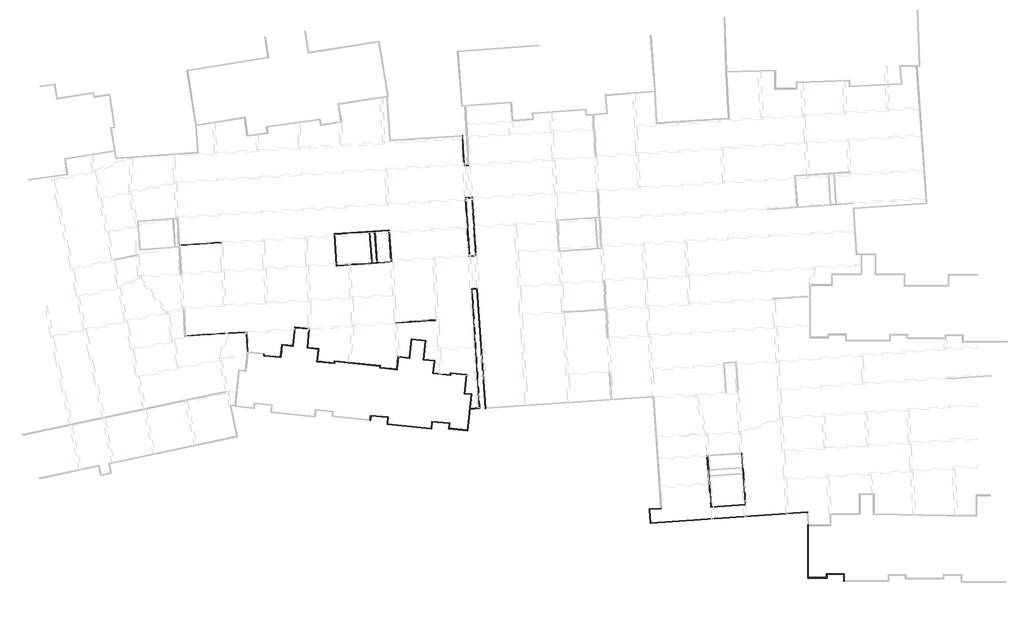
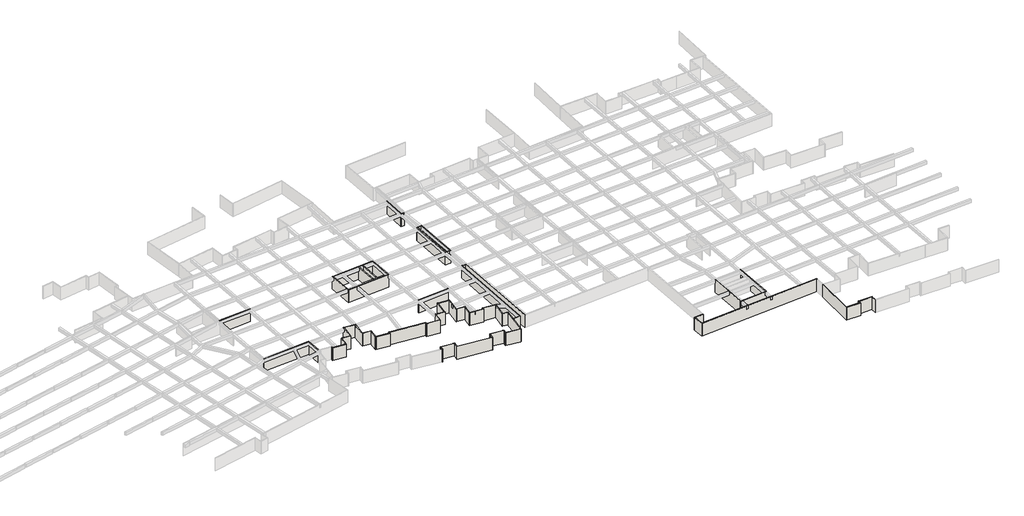
# One storey, part 4 of 14: 66 walls.
"""IFC4 building model written with IfcOpenShell, lengths in millimetres."""

from ifc_helpers import new_model, si_unit, origin, origin_with_axes, place, context, project, spatial, polyline, outline, extrude, faceted_brep, element, save

model = new_model("IFC4")

# Units and contexts
model_context = context("Model", 3, world=origin())
ifc_project = project(units=[si_unit("LENGTHUNIT", "METRE", prefix="MILLI")], contexts=[model_context])

# Site, building, storey
site = spatial("IfcSite", under=ifc_project)
building = spatial("IfcBuilding", under=site)
storey = spatial("IfcBuildingStorey", under=building, Name="户型图", Elevation=0.0)

# Walls
placement = place(None, origin())
element("IfcWall", 1, ObjectType="所有墙体", at=placement, inside=storey, context=model_context, shape_type="Brep", body=[
    faceted_brep([(-177282.9502682, -168363.1803001, 0.0), (-177324.8720819, -168762.0397145, 0.0), (-177324.8720819, -168762.0397145, 3300.0), (-177282.9502682, -168363.1803001, 3300.0), (-177163.6076407, -168375.7237157, 0.0), (-177163.6076407, -168375.7237157, 3300.0), (-177192.765182, -168653.1391901, 3300.0), (-177205.3105083, -168772.4999968, 3300.0), (-177205.3105083, -168772.4999968, 0.0), (-177192.765182, -168653.1391901, 0.0)], [[[0, 1, 2, 3]], [[4, 5, 6, 7, 8, 9]], [[1, 0, 4, 9, 8]], [[3, 2, 7, 6, 5]], [[0, 3, 5, 4]], [[2, 1, 8, 7]]]),
])
element("IfcWall", 2, ObjectType="所有墙体", at=placement, inside=storey, context=model_context, shape_type="Brep", body=[
    faceted_brep([(-177205.3105083, -168772.4999968, 0.0), (-174017.4874744, -169051.3983736, 0.0), (-174017.4874744, -169051.3983736, 3300.0), (-177205.3105083, -168772.4999968, 3300.0), (-177192.765182, -168653.1391901, 0.0), (-177192.765182, -168653.1391901, 3300.0), (-174124.5037217, -168921.5772846, 3300.0), (-174004.9421481, -168932.0375669, 3300.0), (-174004.9421481, -168932.0375669, 0.0), (-174124.5037217, -168921.5772846, 0.0)], [[[0, 1, 2, 3]], [[4, 5, 6, 7, 8, 9]], [[1, 0, 4, 9, 8]], [[3, 2, 7, 6, 5]], [[0, 3, 5, 4]], [[2, 1, 8, 7]]]),
])
element("IfcWall", 3, ObjectType="所有墙体", at=placement, inside=storey, context=model_context, shape_type="Brep", body=[
    faceted_brep([(-174004.9421481, -168932.0375669, 0.0), (-173766.7276803, -166665.5783017, 0.0), (-173754.1842647, -166546.2356743, 0.0), (-173754.1842647, -166546.2356743, 3300.0), (-173766.7276803, -166665.5783017, 3300.0), (-174004.9421481, -168932.0375669, 3300.0), (-174124.5037217, -168921.5772846, 0.0), (-174124.5037217, -168921.5772846, 3300.0), (-173873.5268921, -166533.6922587, 3300.0), (-173873.5268921, -166533.6922587, 0.0)], [[[0, 1, 2, 3, 4, 5]], [[6, 7, 8, 9]], [[2, 1, 0, 6, 9]], [[5, 4, 3, 8, 7]], [[0, 5, 7, 6]], [[3, 2, 9, 8]]]),
])
element("IfcWall", 4, ObjectType="所有墙体", at=placement, inside=storey, context=model_context, shape_type="Brep", body=[
    faceted_brep([(-173766.7276803, -166665.5783017, 0.0), (-171681.9946271, -166884.692575, 0.0), (-171681.9946271, -166884.692575, 3300.0), (-173766.7276803, -166665.5783017, 3300.0), (-173754.1842647, -166546.2356743, 0.0), (-173754.1842647, -166546.2356743, 3300.0), (-171788.7938389, -166752.806532, 3300.0), (-171669.4512115, -166765.3499476, 3300.0), (-171669.4512115, -166765.3499476, 0.0), (-171788.7938389, -166752.806532, 0.0)], [[[0, 1, 2, 3]], [[4, 5, 6, 7, 8, 9]], [[1, 0, 4, 9, 8]], [[3, 2, 7, 6, 5]], [[0, 3, 5, 4]], [[2, 1, 8, 7]]]),
])
element("IfcWall", 5, ObjectType="所有墙体", at=placement, inside=storey, context=model_context, shape_type="Brep", body=[
    faceted_brep([(-171669.4512115, -166765.3499476, 0.0), (-171311.7560707, -163362.1080143, 0.0), (-171299.2126551, -163242.7653869, 0.0), (-171299.2126551, -163242.7653869, 3300.0), (-171311.7560707, -163362.1080143, 3300.0), (-171669.4512115, -166765.3499476, 3300.0), (-171788.7938389, -166752.806532, 0.0), (-171788.7938389, -166752.806532, 3300.0), (-171418.5552825, -163230.2219713, 3300.0), (-171418.5552825, -163230.2219713, 0.0)], [[[0, 1, 2, 3, 4, 5]], [[6, 7, 8, 9]], [[2, 1, 0, 6, 9]], [[5, 4, 3, 8, 7]], [[0, 5, 7, 6]], [[3, 2, 9, 8]]]),
])
element("IfcWall", 6, ObjectType="所有墙体", at=placement, inside=storey, context=model_context, shape_type="Brep", body=[
    faceted_brep([(-171311.7560707, -163362.1080143, 0.0), (-168752.1891607, -163631.129337, 0.0), (-168632.8283541, -163643.6746633, 0.0), (-168632.8283541, -163643.6746633, 3300.0), (-168752.1891607, -163631.129337, 3300.0), (-171311.7560707, -163362.1080143, 3300.0), (-171299.2126551, -163242.7653869, 0.0), (-171299.2126551, -163242.7653869, 3300.0), (-168622.3680718, -163524.1130897, 3300.0), (-168622.3680718, -163524.1130897, 0.0)], [[[0, 1, 2, 3, 4, 5]], [[6, 7, 8, 9]], [[2, 1, 0, 6, 9]], [[5, 4, 3, 8, 7]], [[0, 5, 7, 6]], [[3, 2, 9, 8]]]),
])
element("IfcWall", 7, ObjectType="所有墙体", at=placement, inside=storey, context=model_context, shape_type="Brep", body=[
    faceted_brep([(-168752.1891607, -163631.129337, 0.0), (-169065.9498346, -167217.4302502, 0.0), (-169065.9498346, -167217.4302502, 3300.0), (-168752.1891607, -163631.129337, 3300.0), (-168632.8283541, -163643.6746633, 0.0), (-168632.8283541, -163643.6746633, 3300.0), (-168936.1287457, -167110.4140029, 3300.0), (-168946.589028, -167229.9755765, 3300.0), (-168946.589028, -167229.9755765, 0.0), (-168936.1287457, -167110.4140029, 0.0)], [[[0, 1, 2, 3]], [[4, 5, 6, 7, 8, 9]], [[1, 0, 4, 9, 8]], [[3, 2, 7, 6, 5]], [[0, 3, 5, 4]], [[2, 1, 8, 7]]]),
])
element("IfcWall", 8, ObjectType="所有墙体", at=placement, inside=storey, context=model_context, shape_type="Brep", body=[
    faceted_brep([(-168946.589028, -167229.9755765, 0.0), (-166978.4863314, -167436.8315053, 0.0), (-166859.1437039, -167449.3749209, 0.0), (-166859.1437039, -167449.3749209, 3300.0), (-166978.4863314, -167436.8315053, 3300.0), (-168946.589028, -167229.9755765, 3300.0), (-168936.1287457, -167110.4140029, 0.0), (-168936.1287457, -167110.4140029, 3300.0), (-166846.6002884, -167330.0322935, 3300.0), (-166846.6002884, -167330.0322935, 0.0)], [[[0, 1, 2, 3, 4, 5]], [[6, 7, 8, 9]], [[2, 1, 0, 6, 9]], [[5, 4, 3, 8, 7]], [[0, 5, 7, 6]], [[3, 2, 9, 8]]]),
])
element("IfcWall", 9, ObjectType="所有墙体", at=placement, inside=storey, context=model_context, shape_type="Brep", body=[
    faceted_brep([(-166978.4863314, -167436.8315053, 0.0), (-167229.3546432, -169823.6840542, 0.0), (-167229.3546432, -169823.6840542, 3300.0), (-166978.4863314, -167436.8315053, 3300.0), (-166859.1437039, -167449.3749209, 0.0), (-166859.1437039, -167449.3749209, 3300.0), (-167097.4686002, -169716.8848423, 3300.0), (-167110.0120158, -169836.2274698, 3300.0), (-167110.0120158, -169836.2274698, 0.0), (-167097.4686002, -169716.8848423, 0.0)], [[[0, 1, 2, 3]], [[4, 5, 6, 7, 8, 9]], [[1, 0, 4, 9, 8]], [[3, 2, 7, 6, 5]], [[0, 3, 5, 4]], [[2, 1, 8, 7]]]),
])
element("IfcWall", 10, ObjectType="所有墙体", at=placement, inside=storey, context=model_context, shape_type="Brep", body=[
    faceted_brep([(-167110.0120158, -169836.2274698, 0.0), (-163828.0897611, -170181.1713986, 0.0), (-163828.0897611, -170181.1713986, 3300.0), (-167110.0120158, -169836.2274698, 3300.0), (-167097.4686002, -169716.8848423, 0.0), (-167097.4686002, -169716.8848423, 3300.0), (-163934.8889729, -170049.2853555, 3300.0), (-163815.5463455, -170061.8287711, 3300.0), (-163815.5463455, -170061.8287711, 0.0), (-163934.8889729, -170049.2853555, 0.0)], [[[0, 1, 2, 3]], [[4, 5, 6, 7, 8, 9]], [[1, 0, 4, 9, 8]], [[3, 2, 7, 6, 5]], [[0, 3, 5, 4]], [[2, 1, 8, 7]]]),
])
element("IfcWall", 11, ObjectType="所有墙体", at=placement, inside=storey, context=model_context, shape_type="Brep", body=[
    faceted_brep([(-163815.5463455, -170061.8287711, 0.0), (-163786.2783758, -169783.3626404, 0.0), (-163773.7349602, -169664.020013, 0.0), (-163773.7349602, -169664.020013, 3300.0), (-163786.2783758, -169783.3626404, 3300.0), (-163815.5463455, -170061.8287711, 3300.0), (-163934.8889729, -170049.2853555, 0.0), (-163934.8889729, -170049.2853555, 3300.0), (-163893.0775876, -169651.4765974, 3300.0), (-163893.0775876, -169651.4765974, 0.0)], [[[0, 1, 2, 3, 4, 5]], [[6, 7, 8, 9]], [[2, 1, 0, 6, 9]], [[5, 4, 3, 8, 7]], [[0, 5, 7, 6]], [[3, 2, 9, 8]]]),
])
element("IfcWall", 12, ObjectType="所有墙体", at=placement, inside=storey, context=model_context, shape_type="Brep", body=[
    faceted_brep([(-163786.2783758, -169783.3626404, 0.0), (-155253.2805135, -170680.2168553, 0.0), (-155133.9378861, -170692.7602708, 0.0), (-155133.9378861, -170692.7602708, 3300.0), (-155253.2805135, -170680.2168553, 3300.0), (-163786.2783758, -169783.3626404, 3300.0), (-163773.7349602, -169664.020013, 0.0), (-163773.7349602, -169664.020013, 3300.0), (-155121.3944705, -170573.4176434, 3300.0), (-155121.3944705, -170573.4176434, 0.0)], [[[0, 1, 2, 3, 4, 5]], [[6, 7, 8, 9]], [[2, 1, 0, 6, 9]], [[5, 4, 3, 8, 7]], [[0, 5, 7, 6]], [[3, 2, 9, 8]]]),
])
element("IfcWall", 13, ObjectType="所有墙体", at=placement, inside=storey, context=model_context, shape_type="Brep", body=[
    faceted_brep([(-155253.2805135, -170680.2168553, 0.0), (-155286.7296218, -170998.4638618, 0.0), (-155286.7296218, -170998.4638618, 3300.0), (-155253.2805135, -170680.2168553, 3300.0), (-155133.9378861, -170692.7602708, 0.0), (-155133.9378861, -170692.7602708, 3300.0), (-155154.8435787, -170891.6646499, 3300.0), (-155167.3869943, -171011.0072774, 3300.0), (-155167.3869943, -171011.0072774, 0.0), (-155154.8435787, -170891.6646499, 0.0)], [[[0, 1, 2, 3]], [[4, 5, 6, 7, 8, 9]], [[1, 0, 4, 9, 8]], [[3, 2, 7, 6, 5]], [[0, 3, 5, 4]], [[2, 1, 8, 7]]]),
])
element("IfcWall", 14, ObjectType="所有墙体", at=placement, inside=storey, context=model_context, shape_type="Brep", body=[
    faceted_brep([(-155167.3869943, -171011.0072774, 0.0), (-151965.0264912, -171347.5889291, 0.0), (-151965.0264912, -171347.5889291, 3300.0), (-155167.3869943, -171011.0072774, 3300.0), (-155154.8435787, -170891.6646499, 0.0), (-155154.8435787, -170891.6646499, 3300.0), (-152071.8257031, -171215.702886, 3300.0), (-151952.4830756, -171228.2463016, 3300.0), (-151952.4830756, -171228.2463016, 0.0), (-152071.8257031, -171215.702886, 0.0)], [[[0, 1, 2, 3]], [[4, 5, 6, 7, 8, 9]], [[1, 0, 4, 9, 8]], [[3, 2, 7, 6, 5]], [[0, 3, 5, 4]], [[2, 1, 8, 7]]]),
])
element("IfcWall", 15, ObjectType="所有墙体", at=placement, inside=storey, context=model_context, shape_type="Brep", body=[
    faceted_brep([(-151952.4830756, -171228.2463016, 0.0), (-151714.1581794, -168960.7363802, 0.0), (-151701.6147638, -168841.3937528, 0.0), (-151701.6147638, -168841.3937528, 3300.0), (-151714.1581794, -168960.7363802, 3300.0), (-151952.4830756, -171228.2463016, 3300.0), (-152071.8257031, -171215.702886, 0.0), (-152071.8257031, -171215.702886, 3300.0), (-151820.9573912, -168828.8503372, 3300.0), (-151820.9573912, -168828.8503372, 0.0)], [[[0, 1, 2, 3, 4, 5]], [[6, 7, 8, 9]], [[2, 1, 0, 6, 9]], [[5, 4, 3, 8, 7]], [[0, 5, 7, 6]], [[3, 2, 9, 8]]]),
])
element("IfcWall", 16, ObjectType="所有墙体", at=placement, inside=storey, context=model_context, shape_type="Brep", body=[
    faceted_brep([(-151714.1581794, -168960.7363802, 0.0), (-149565.9908854, -169186.5178609, 0.0), (-149565.9908854, -169186.5178609, 3300.0), (-151714.1581794, -168960.7363802, 3300.0), (-151701.6147638, -168841.3937528, 0.0), (-151701.6147638, -168841.3937528, 3300.0), (-149672.7900972, -169054.6318178, 3300.0), (-149553.4474698, -169067.1752334, 3300.0), (-149553.4474698, -169067.1752334, 0.0), (-149672.7900972, -169054.6318178, 0.0)], [[[0, 1, 2, 3]], [[4, 5, 6, 7, 8, 9]], [[1, 0, 4, 9, 8]], [[3, 2, 7, 6, 5]], [[0, 3, 5, 4]], [[2, 1, 8, 7]]]),
])
element("IfcWall", 17, ObjectType="所有墙体", at=placement, inside=storey, context=model_context, shape_type="Brep", body=[
    faceted_brep([(-149553.4474698, -169067.1752334, 0.0), (-149188.039961, -165590.5550201, 0.0), (-149175.4965454, -165471.2123926, 0.0), (-149175.4965454, -165471.2123926, 3300.0), (-149188.039961, -165590.5550201, 3300.0), (-149553.4474698, -169067.1752334, 3300.0), (-149672.7900972, -169054.6318178, 0.0), (-149672.7900972, -169054.6318178, 3300.0), (-149294.8391728, -165458.668977, 3300.0), (-149294.8391728, -165458.668977, 0.0)], [[[0, 1, 2, 3, 4, 5]], [[6, 7, 8, 9]], [[2, 1, 0, 6, 9]], [[5, 4, 3, 8, 7]], [[0, 5, 7, 6]], [[3, 2, 9, 8]]]),
])
element("IfcWall", 18, ObjectType="所有墙体", at=placement, inside=storey, context=model_context, shape_type="Brep", body=[
    faceted_brep([(-149188.039961, -165590.5550201, 0.0), (-146615.1929513, -165860.9721375, 0.0), (-146495.8503238, -165873.5155531, 0.0), (-146495.8503238, -165873.5155531, 3300.0), (-146615.1929513, -165860.9721375, 3300.0), (-149188.039961, -165590.5550201, 3300.0), (-149175.4965454, -165471.2123926, 0.0), (-149175.4965454, -165471.2123926, 3300.0), (-146483.3069082, -165754.1729256, 3300.0), (-146483.3069082, -165754.1729256, 0.0)], [[[0, 1, 2, 3, 4, 5]], [[6, 7, 8, 9]], [[2, 1, 0, 6, 9]], [[5, 4, 3, 8, 7]], [[0, 5, 7, 6]], [[3, 2, 9, 8]]]),
])
element("IfcWall", 19, ObjectType="所有墙体", at=placement, inside=storey, context=model_context, shape_type="Brep", body=[
    faceted_brep([(-146615.1929513, -165860.9721375, 0.0), (-146993.1438757, -169456.9349783, 0.0), (-146993.1438757, -169456.9349783, 3300.0), (-146615.1929513, -165860.9721375, 3300.0), (-146495.8503238, -165873.5155531, 0.0), (-146495.8503238, -165873.5155531, 3300.0), (-146861.2578327, -169350.1357664, 3300.0), (-146873.8012483, -169469.4783939, 3300.0), (-146873.8012483, -169469.4783939, 0.0), (-146861.2578327, -169350.1357664, 0.0)], [[[0, 1, 2, 3]], [[4, 5, 6, 7, 8, 9]], [[1, 0, 4, 9, 8]], [[3, 2, 7, 6, 5]], [[0, 3, 5, 4]], [[2, 1, 8, 7]]]),
])
element("IfcWall", 20, ObjectType="所有墙体", at=placement, inside=storey, context=model_context, shape_type="Brep", body=[
    faceted_brep([(-146873.8012483, -169469.4783939, 0.0), (-144944.4287712, -169672.2636126, 0.0), (-144825.0861438, -169684.8070282, 0.0), (-144825.0861438, -169684.8070282, 3300.0), (-144944.4287712, -169672.2636126, 3300.0), (-146873.8012483, -169469.4783939, 3300.0), (-146861.2578327, -169350.1357664, 0.0), (-146861.2578327, -169350.1357664, 3300.0), (-144812.5427282, -169565.4644007, 3300.0), (-144812.5427282, -169565.4644007, 0.0)], [[[0, 1, 2, 3, 4, 5]], [[6, 7, 8, 9]], [[2, 1, 0, 6, 9]], [[5, 4, 3, 8, 7]], [[0, 5, 7, 6]], [[3, 2, 9, 8]]]),
])
element("IfcWall", 21, ObjectType="所有墙体", at=placement, inside=storey, context=model_context, shape_type="Brep", body=[
    faceted_brep([(-144944.4287712, -169672.2636126, 0.0), (-145197.8384373, -172083.2955318, 0.0), (-145197.8384373, -172083.2955318, 3300.0), (-144944.4287712, -169672.2636126, 3300.0), (-144825.0861438, -169684.8070282, 0.0), (-144825.0861438, -169684.8070282, 3300.0), (-145065.9523943, -171976.49632, 3300.0), (-145078.4958099, -172095.8389474, 3300.0), (-145078.4958099, -172095.8389474, 0.0), (-145065.9523943, -171976.49632, 0.0)], [[[0, 1, 2, 3]], [[4, 5, 6, 7, 8, 9]], [[1, 0, 4, 9, 8]], [[3, 2, 7, 6, 5]], [[0, 3, 5, 4]], [[2, 1, 8, 7]]]),
])
element("IfcWall", 22, ObjectType="所有墙体", at=placement, inside=storey, context=model_context, shape_type="Brep", body=[
    faceted_brep([(-145078.4958099, -172095.8389474, 0.0), (-141793.9940812, -172441.0539898, 0.0), (-141793.9940812, -172441.0539898, 3300.0), (-145078.4958099, -172095.8389474, 3300.0), (-145065.9523943, -171976.49632, 0.0), (-145065.9523943, -171976.49632, 3300.0), (-141900.793293, -172309.1679468, 3300.0), (-141781.4506656, -172321.7113624, 3300.0), (-141781.4506656, -172321.7113624, 0.0), (-141900.793293, -172309.1679468, 0.0)], [[[0, 1, 2, 3]], [[4, 5, 6, 7, 8, 9]], [[1, 0, 4, 9, 8]], [[3, 2, 7, 6, 5]], [[0, 3, 5, 4]], [[2, 1, 8, 7]]]),
])
element("IfcWall", 23, ObjectType="所有墙体", at=placement, inside=storey, context=model_context, shape_type="Brep", body=[
    faceted_brep([(-141781.4506656, -172321.7113624, 0.0), (-141752.1826958, -172043.2452317, 0.0), (-141739.6392803, -171923.9026042, 0.0), (-141739.6392803, -171923.9026042, 3300.0), (-141752.1826958, -172043.2452317, 3300.0), (-141781.4506656, -172321.7113624, 3300.0), (-141900.793293, -172309.1679468, 0.0), (-141900.793293, -172309.1679468, 3300.0), (-141858.9819077, -171911.3591887, 3300.0), (-141858.9819077, -171911.3591887, 0.0)], [[[0, 1, 2, 3, 4, 5]], [[6, 7, 8, 9]], [[2, 1, 0, 6, 9]], [[5, 4, 3, 8, 7]], [[0, 5, 7, 6]], [[3, 2, 9, 8]]]),
])
element("IfcWall", 24, ObjectType="所有墙体", at=placement, inside=storey, context=model_context, shape_type="Brep", body=[
    faceted_brep([(-141752.1826958, -172043.2452317, 0.0), (-138848.6738606, -172348.4163074, 0.0), (-138729.3312331, -172360.959723, 0.0), (-138729.3312331, -172360.959723, 3300.0), (-138848.6738606, -172348.4163074, 3300.0), (-141752.1826958, -172043.2452317, 3300.0), (-141739.6392803, -171923.9026042, 0.0), (-141739.6392803, -171923.9026042, 3300.0), (-138716.7878176, -172241.6170956, 3300.0), (-138716.7878176, -172241.6170956, 0.0)], [[[0, 1, 2, 3, 4, 5]], [[6, 7, 8, 9]], [[2, 1, 0, 6, 9]], [[5, 4, 3, 8, 7]], [[0, 5, 7, 6]], [[3, 2, 9, 8]]]),
])
element("IfcWall", 25, ObjectType="所有墙体", at=placement, inside=storey, context=model_context, shape_type="Brep", body=[
    faceted_brep([(-138848.6738606, -172348.4163074, 0.0), (-139223.583115, -175915.4395908, 0.0), (-139223.583115, -175915.4395908, 3300.0), (-138848.6738606, -172348.4163074, 3300.0), (-138729.3312331, -172360.959723, 0.0), (-138729.3312331, -172360.959723, 3300.0), (-139091.6970719, -175808.640379, 3300.0), (-139104.2404875, -175927.9830064, 3300.0), (-139104.2404875, -175927.9830064, 0.0), (-139091.6970719, -175808.640379, 0.0)], [[[0, 1, 2, 3]], [[4, 5, 6, 7, 8, 9]], [[1, 0, 4, 9, 8]], [[3, 2, 7, 6, 5]], [[0, 3, 5, 4]], [[2, 1, 8, 7]]]),
])
element("IfcWall", 26, ObjectType="所有墙体", at=placement, inside=storey, context=model_context, shape_type="Brep", body=[
    faceted_brep([(-139104.2404875, -175927.9830064, 0.0), (-137913.6531673, -176053.1187762, 0.0), (-137794.3105398, -176065.6621918, 0.0), (-137794.3105398, -176065.6621918, 3300.0), (-137913.6531673, -176053.1187762, 3300.0), (-139104.2404875, -175927.9830064, 3300.0), (-139091.6970719, -175808.640379, 0.0), (-139091.6970719, -175808.640379, 3300.0), (-137781.7671242, -175946.3195644, 3300.0), (-137781.7671242, -175946.3195644, 0.0)], [[[0, 1, 2, 3, 4, 5]], [[6, 7, 8, 9]], [[2, 1, 0, 6, 9]], [[5, 4, 3, 8, 7]], [[0, 5, 7, 6]], [[3, 2, 9, 8]]]),
])
element("IfcWall", 27, ObjectType="所有墙体", at=placement, inside=storey, context=model_context, shape_type="Brep", body=[
    faceted_brep([(-137913.6531673, -176053.1187762, 0.0), (-138624.4467175, -182815.8676647, 0.0), (-138636.9901331, -182935.2102922, 0.0), (-138636.9901331, -182935.2102922, 3300.0), (-138624.4467175, -182815.8676647, 3300.0), (-137913.6531673, -176053.1187762, 3300.0), (-137794.3105398, -176065.6621918, 0.0), (-137794.3105398, -176065.6621918, 3300.0), (-138073.1042952, -178718.2075878, 3300.0), (-138085.9279381, -178840.2164005, 3300.0), (-138517.6475056, -182947.7537078, 3300.0), (-138517.6475056, -182947.7537078, 0.0), (-138085.9279381, -178840.2164005, 0.0), (-138073.1042952, -178718.2075878, 0.0)], [[[0, 1, 2, 3, 4, 5]], [[6, 7, 8, 9, 10, 11, 12, 13]], [[2, 1, 0, 6, 13, 12, 11]], [[5, 4, 3, 10, 9, 8, 7]], [[0, 5, 7, 6]], [[3, 2, 11, 10]]]),
])
element("IfcWall", 28, ObjectType="所有墙体", at=placement, inside=storey, context=model_context, shape_type="Brep", body=[
    faceted_brep([(-138624.4467175, -182815.8676647, 0.0), (-142085.3829134, -182452.1086125, 0.0), (-142204.7255408, -182439.565197, 0.0), (-142204.7255408, -182439.565197, 3300.0), (-142085.3829134, -182452.1086125, 3300.0), (-138624.4467175, -182815.8676647, 3300.0), (-138636.9901331, -182935.2102922, 0.0), (-138636.9901331, -182935.2102922, 3300.0), (-142217.2689564, -182558.9078244, 3300.0), (-142217.2689564, -182558.9078244, 0.0)], [[[0, 1, 2, 3, 4, 5]], [[6, 7, 8, 9]], [[2, 1, 0, 6, 9]], [[5, 4, 3, 8, 7]], [[0, 5, 7, 6]], [[3, 2, 9, 8]]]),
])
element("IfcWall", 29, ObjectType="所有墙体", at=placement, inside=storey, context=model_context, shape_type="Brep", body=[
    faceted_brep([(-142085.3829134, -182452.1086125, 0.0), (-141982.9450194, -181477.4771551, 0.0), (-141982.9450194, -181477.4771551, 3300.0), (-142085.3829134, -182452.1086125, 3300.0), (-142204.7255408, -182439.565197, 0.0), (-142204.7255408, -182439.565197, 3300.0), (-142114.8310624, -181584.2763669, 3300.0), (-142102.2876468, -181464.9337395, 3300.0), (-142102.2876468, -181464.9337395, 0.0), (-142114.8310624, -181584.2763669, 0.0)], [[[0, 1, 2, 3]], [[4, 5, 6, 7, 8, 9]], [[1, 0, 4, 9, 8]], [[3, 2, 7, 6, 5]], [[0, 3, 5, 4]], [[2, 1, 8, 7]]]),
])
element("IfcWall", 30, ObjectType="所有墙体", at=placement, inside=storey, context=model_context, shape_type="Brep", body=[
    faceted_brep([(-142102.2876468, -181464.9337395, 0.0), (-145371.9189814, -181121.2816385, 0.0), (-145371.9189814, -181121.2816385, 3300.0), (-142102.2876468, -181464.9337395, 3300.0), (-142114.8310624, -181584.2763669, 0.0), (-142114.8310624, -181584.2763669, 3300.0), (-145265.1197696, -181253.1676815, 3300.0), (-145384.462397, -181240.6242659, 3300.0), (-145384.462397, -181240.6242659, 0.0), (-145265.1197696, -181253.1676815, 0.0)], [[[0, 1, 2, 3]], [[4, 5, 6, 7, 8, 9]], [[1, 0, 4, 9, 8]], [[3, 2, 7, 6, 5]], [[0, 3, 5, 4]], [[2, 1, 8, 7]]]),
])
element("IfcWall", 31, ObjectType="所有墙体", at=placement, inside=storey, context=model_context, shape_type="Brep", body=[
    faceted_brep([(-145384.462397, -181240.6242659, 0.0), (-145515.3052758, -182485.5111007, 0.0), (-145527.8486914, -182604.8537281, 0.0), (-145527.8486914, -182604.8537281, 3300.0), (-145515.3052758, -182485.5111007, 3300.0), (-145384.462397, -181240.6242659, 3300.0), (-145265.1197696, -181253.1676815, 0.0), (-145265.1197696, -181253.1676815, 3300.0), (-145408.5060639, -182617.3971437, 3300.0), (-145408.5060639, -182617.3971437, 0.0)], [[[0, 1, 2, 3, 4, 5]], [[6, 7, 8, 9]], [[2, 1, 0, 6, 9]], [[5, 4, 3, 8, 7]], [[0, 5, 7, 6]], [[3, 2, 9, 8]]]),
])
element("IfcWall", 32, ObjectType="所有墙体", at=placement, inside=storey, context=model_context, shape_type="Brep", body=[
    faceted_brep([(-145515.3052758, -182485.5111007, 0.0), (-153747.1228731, -181620.3122073, 0.0), (-153866.4655006, -181607.7687917, 0.0), (-153866.4655006, -181607.7687917, 3300.0), (-153747.1228731, -181620.3122073, 3300.0), (-145515.3052758, -182485.5111007, 3300.0), (-145527.8486914, -182604.8537281, 0.0), (-145527.8486914, -182604.8537281, 3300.0), (-153879.0089162, -181727.1114191, 3300.0), (-153879.0089162, -181727.1114191, 0.0)], [[[0, 1, 2, 3, 4, 5]], [[6, 7, 8, 9]], [[2, 1, 0, 6, 9]], [[5, 4, 3, 8, 7]], [[0, 5, 7, 6]], [[3, 2, 9, 8]]]),
])
element("IfcWall", 33, ObjectType="所有墙体", at=placement, inside=storey, context=model_context, shape_type="Brep", body=[
    faceted_brep([(-153747.1228731, -181620.3122073, 0.0), (-153613.0639979, -180344.8272098, 0.0), (-153613.0639979, -180344.8272098, 3300.0), (-153747.1228731, -181620.3122073, 3300.0), (-153866.4655006, -181607.7687917, 0.0), (-153866.4655006, -181607.7687917, 3300.0), (-153744.9500409, -180451.6264217, 3300.0), (-153732.4066253, -180332.2837942, 3300.0), (-153732.4066253, -180332.2837942, 0.0), (-153744.9500409, -180451.6264217, 0.0)], [[[0, 1, 2, 3]], [[4, 5, 6, 7, 8, 9]], [[1, 0, 4, 9, 8]], [[3, 2, 7, 6, 5]], [[0, 3, 5, 4]], [[2, 1, 8, 7]]]),
])
element("IfcWall", 34, ObjectType="所有墙体", at=placement, inside=storey, context=model_context, shape_type="Brep", body=[
    faceted_brep([(-153732.4066253, -180332.2837942, 0.0), (-157016.9929588, -179987.0598595, 0.0), (-157016.9929588, -179987.0598595, 3300.0), (-153732.4066253, -180332.2837942, 3300.0), (-153744.9500409, -180451.6264217, 0.0), (-153744.9500409, -180451.6264217, 3300.0), (-156910.193747, -180118.9459025, 3300.0), (-157029.5363744, -180106.4024869, 3300.0), (-157029.5363744, -180106.4024869, 0.0), (-156910.193747, -180118.9459025, 0.0)], [[[0, 1, 2, 3]], [[4, 5, 6, 7, 8, 9]], [[1, 0, 4, 9, 8]], [[3, 2, 7, 6, 5]], [[0, 3, 5, 4]], [[2, 1, 8, 7]]]),
])
element("IfcWall", 35, ObjectType="所有墙体", at=placement, inside=storey, context=model_context, shape_type="Brep", body=[
    faceted_brep([(-157029.5363744, -180106.4024869, 0.0), (-157110.1034337, -180872.9468522, 0.0), (-157122.6468493, -180992.2894796, 0.0), (-157122.6468493, -180992.2894796, 3300.0), (-157110.1034337, -180872.9468522, 3300.0), (-157029.5363744, -180106.4024869, 3300.0), (-156910.193747, -180118.9459025, 0.0), (-156910.193747, -180118.9459025, 3300.0), (-157003.3042219, -181004.8328952, 3300.0), (-157003.3042219, -181004.8328952, 0.0)], [[[0, 1, 2, 3, 4, 5]], [[6, 7, 8, 9]], [[2, 1, 0, 6, 9]], [[5, 4, 3, 8, 7]], [[0, 5, 7, 6]], [[3, 2, 9, 8]]]),
])
element("IfcWall", 36, ObjectType="所有墙体", at=placement, inside=storey, context=model_context, shape_type="Brep", body=[
    faceted_brep([(-73965.252881, -200843.9572436, 0.0), (-73965.252881, -210934.2549962, 0.0), (-73965.252881, -210934.2549962, 3300.0), (-73965.252881, -200843.9572436, 3300.0), (-73845.252881, -200843.9572436, 0.0), (-73845.252881, -200843.9572436, 3300.0), (-73845.252881, -200963.9572436, 3300.0), (-73845.252881, -210814.2549962, 3300.0), (-73845.252881, -210934.2549962, 3300.0), (-73845.252881, -210934.2549962, 0.0), (-73845.252881, -210814.2549962, 0.0), (-73845.252881, -200963.9572436, 0.0), (-73914.792994, -200843.9572436, 0.0), (-73914.792994, -200843.9572436, 3300.0)], [[[0, 1, 2, 3]], [[4, 5, 6, 7, 8, 9, 10, 11]], [[1, 0, 12, 4, 11, 10, 9]], [[3, 2, 8, 7, 6, 5, 13]], [[2, 1, 9, 8]], [[0, 3, 13, 5, 4, 12]]]),
])
element("IfcWall", 37, ObjectType="所有墙体", at=placement, inside=storey, context=model_context, shape_type="Brep", body=[
    faceted_brep([(-73845.252881, -210934.2549962, 0.0), (-70315.6322741, -210934.2549962, 0.0), (-70315.6322741, -210934.2549962, 3300.0), (-73845.252881, -210934.2549962, 3300.0), (-73845.252881, -210814.2549962, 0.0), (-73845.252881, -210814.2549962, 3300.0), (-70435.6322741, -210814.2549962, 3300.0), (-70315.6322741, -210814.2549962, 3300.0), (-70315.6322741, -210814.2549962, 0.0), (-70435.6322741, -210814.2549962, 0.0)], [[[0, 1, 2, 3]], [[4, 5, 6, 7, 8, 9]], [[1, 0, 4, 9, 8]], [[3, 2, 7, 6, 5]], [[0, 3, 5, 4]], [[2, 1, 8, 7]]]),
])
element("IfcWall", 38, ObjectType="所有墙体", at=placement, inside=storey, context=model_context, shape_type="Brep", body=[
    faceted_brep([(-70315.6322741, -210814.2549962, 0.0), (-70315.6322741, -210259.3587102, 0.0), (-70315.6322741, -210139.3587102, 0.0), (-70315.6322741, -210139.3587102, 3300.0), (-70315.6322741, -210259.3587102, 3300.0), (-70315.6322741, -210814.2549962, 3300.0), (-70435.6322741, -210814.2549962, 0.0), (-70435.6322741, -210814.2549962, 3300.0), (-70435.6322741, -210139.3587102, 3300.0), (-70435.6322741, -210139.3587102, 0.0)], [[[0, 1, 2, 3, 4, 5]], [[6, 7, 8, 9]], [[2, 1, 0, 6, 9]], [[5, 4, 3, 8, 7]], [[0, 5, 7, 6]], [[3, 2, 9, 8]]]),
])
element("IfcWall", 39, ObjectType="所有墙体", at=placement, inside=storey, context=model_context, shape_type="Brep", body=[
    faceted_brep([(-70315.6322741, -210259.3587102, 0.0), (-67130.794427, -210259.3587102, 0.0), (-67010.794427, -210259.3587102, 0.0), (-67010.794427, -210259.3587102, 3300.0), (-67130.794427, -210259.3587102, 3300.0), (-70315.6322741, -210259.3587102, 3300.0), (-70315.6322741, -210139.3587102, 0.0), (-70315.6322741, -210139.3587102, 3300.0), (-67010.794427, -210139.3587102, 3300.0), (-67010.794427, -210139.3587102, 0.0)], [[[0, 1, 2, 3, 4, 5]], [[6, 7, 8, 9]], [[2, 1, 0, 6, 9]], [[5, 4, 3, 8, 7]], [[0, 5, 7, 6]], [[3, 2, 9, 8]]]),
])
element("IfcWall", 40, ObjectType="所有墙体", at=placement, inside=storey, context=model_context, shape_type="Brep", body=[
    faceted_brep([(-67130.794427, -210259.3587102, 0.0), (-67130.794427, -211582.679776, 0.0), (-67130.794427, -211582.679776, 3300.0), (-67130.794427, -210259.3587102, 3300.0), (-67010.794427, -210259.3587102, 0.0), (-67010.794427, -210259.3587102, 3300.0), (-67010.794427, -211462.679776, 3300.0), (-67010.794427, -211582.679776, 3300.0), (-67010.794427, -211582.679776, 0.0), (-67010.794427, -211462.679776, 0.0)], [[[0, 1, 2, 3]], [[4, 5, 6, 7, 8, 9]], [[1, 0, 4, 9, 8]], [[3, 2, 7, 6, 5]], [[0, 3, 5, 4]], [[2, 1, 8, 7]]]),
])
element("IfcWall", 41, ObjectType="所有墙体", at=placement, inside=storey, context=model_context, shape_type="Brep", body=[
    faceted_brep([(-138085.9279381, -178840.2164005, 0.0), (-136287.0596037, -178651.1477199, 0.0), (-136287.0596037, -178651.1477199, 3300.0), (-138085.9279381, -178840.2164005, 3300.0), (-138073.1042952, -178718.2075878, 0.0), (-138073.1042952, -178718.2075878, 3300.0), (-136413.702619, -178543.7974436, 3300.0), (-136294.2395296, -178531.241367, 3300.0), (-136294.2395296, -178531.241367, 0.0), (-136413.702619, -178543.7974436, 0.0)], [[[0, 1, 2, 3]], [[4, 5, 6, 7, 8, 9]], [[1, 0, 4, 9, 8]], [[3, 2, 7, 6, 5]], [[0, 3, 5, 4]], [[2, 1, 8, 7]]]),
])
element("IfcWall", 42, ObjectType="所有墙体", at=placement, inside=storey, context=model_context, shape_type="Brep", body=[
    faceted_brep([(-136294.2395296, -178531.241367, 0.0), (-137643.5139612, -155998.059439, 0.0), (-137650.6994946, -155878.059439, 0.0), (-137650.6994946, -155878.059439, 3300.0), (-137643.5139612, -155998.059439, 3300.0), (-136294.2395296, -178531.241367, 3300.0), (-136413.702619, -178543.7974436, 0.0), (-136413.702619, -178543.7974436, 3300.0), (-137770.914435, -155878.059439, 3300.0), (-137770.914435, -155878.059439, 0.0)], [[[0, 1, 2, 3, 4, 5]], [[6, 7, 8, 9]], [[2, 1, 0, 6, 9]], [[5, 4, 3, 8, 7]], [[0, 5, 7, 6]], [[3, 2, 9, 8]]]),
])
element("IfcWall", 43, ObjectType="所有墙体", at=placement, inside=storey, context=model_context, shape_type="Brep", body=[
    faceted_brep([(-137643.5139612, -155998.059439, 0.0), (-136863.1651032, -155998.059439, 0.0), (-136742.8720755, -155998.059439, 0.0), (-136742.8720755, -155998.059439, 3300.0), (-136863.1651032, -155998.059439, 3300.0), (-137643.5139612, -155998.059439, 3300.0), (-137650.6994946, -155878.059439, 0.0), (-137650.6994946, -155878.059439, 3300.0), (-136751.2632929, -155878.059439, 3300.0), (-136751.2632929, -155878.059439, 0.0)], [[[0, 1, 2, 3, 4, 5]], [[6, 7, 8, 9]], [[2, 1, 0, 6, 9]], [[5, 4, 3, 8, 7]], [[0, 5, 7, 6]], [[3, 2, 9, 8]]]),
])
element("IfcWall", 44, ObjectType="所有墙体", at=placement, inside=storey, context=model_context, shape_type="Brep", body=[
    faceted_brep([(-136863.1651032, -155998.059439, 0.0), (-135272.4350513, -178746.5590164, 0.0), (-135272.4350513, -178746.5590164, 3300.0), (-136863.1651032, -155998.059439, 3300.0), (-136742.8720755, -155998.059439, 0.0), (-136742.8720755, -155998.059439, 3300.0), (-135161.0981421, -178618.4805535, 3300.0), (-135152.7273653, -178738.1882395, 3300.0), (-135152.7273653, -178738.1882395, 0.0), (-135161.0981421, -178618.4805535, 0.0)], [[[0, 1, 2, 3]], [[4, 5, 6, 7, 8, 9]], [[1, 0, 4, 9, 8]], [[3, 2, 7, 6, 5]], [[0, 3, 5, 4]], [[2, 1, 8, 7]]]),
])
element("IfcWall", 45, ObjectType="所有墙体", at=placement, inside=storey, context=model_context, shape_type="Brep", body=[
    faceted_brep([(-101872.9433291, -197642.758441, 0.0), (-104100.7618774, -197798.5426897, 0.0), (-104100.7618774, -197798.5426897, 3300.0), (-101872.9433291, -197642.758441, 3300.0), (-101864.5725522, -197762.4661271, 0.0), (-101864.5725522, -197762.4661271, 3300.0), (-103972.6834145, -197909.8795989, 3300.0), (-104092.3911006, -197918.2503757, 3300.0), (-104092.3911006, -197918.2503757, 0.0), (-103972.6834145, -197909.8795989, 0.0)], [[[0, 1, 2, 3]], [[4, 5, 6, 7, 8, 9]], [[1, 0, 4, 9, 8]], [[3, 2, 7, 6, 5]], [[0, 3, 5, 4]], [[2, 1, 8, 7]]]),
])
element("IfcWall", 46, ObjectType="所有墙体", at=placement, inside=storey, context=model_context, shape_type="Brep", body=[
    faceted_brep([(-104092.3911006, -197918.2503757, 0.0), (-103906.4583034, -200577.2132551, 0.0), (-103906.4583034, -200577.2132551, 3300.0), (-104092.3911006, -197918.2503757, 3300.0), (-103972.6834145, -197909.8795989, 0.0), (-103972.6834145, -197909.8795989, 3300.0), (-103795.1213942, -200449.1347922, 3300.0), (-103786.7506173, -200568.8424782, 3300.0), (-103786.7506173, -200568.8424782, 0.0), (-103795.1213942, -200449.1347922, 0.0)], [[[0, 1, 2, 3]], [[4, 5, 6, 7, 8, 9]], [[1, 0, 4, 9, 8]], [[3, 2, 7, 6, 5]], [[0, 3, 5, 4]], [[2, 1, 8, 7]]]),
])
element("IfcWall", 47, ObjectType="所有墙体", at=placement, inside=storey, context=model_context, shape_type="Brep", body=[
    faceted_brep([(-103786.7506173, -200568.8424782, 0.0), (-74079.2932006, -198491.4946901, 0.0), (-73959.5855146, -198483.1239133, 0.0), (-73959.5855146, -198483.1239133, 3300.0), (-74079.2932006, -198491.4946901, 3300.0), (-103786.7506173, -200568.8424782, 3300.0), (-103795.1213942, -200449.1347922, 0.0), (-103795.1213942, -200449.1347922, 3300.0), (-73967.9562914, -198363.4162272, 3300.0), (-73967.9562914, -198363.4162272, 0.0)], [[[0, 1, 2, 3, 4, 5]], [[6, 7, 8, 9]], [[2, 1, 0, 6, 9]], [[5, 4, 3, 8, 7]], [[0, 5, 7, 6]], [[3, 2, 9, 8]]]),
])
element("IfcWall", 48, ObjectType="所有墙体", at=placement, inside=storey, context=model_context, shape_type="Brep", body=[
    faceted_brep([(-138496.8707175, -132411.9487341, 0.0), (-139215.8839825, -132449.6306226, 0.0), (-139335.7195267, -132455.9109373, 0.0), (-139335.7195267, -132455.9109373, 3300.0), (-139215.8839825, -132449.6306226, 3300.0), (-138496.8707175, -132411.9487341, 3300.0), (-138490.5904027, -132531.7842783, 0.0), (-138490.5904027, -132531.7842783, 3300.0), (-139329.4392119, -132575.7464815, 3300.0), (-139329.4392119, -132575.7464815, 0.0)], [[[0, 1, 2, 3, 4, 5]], [[6, 7, 8, 9]], [[2, 1, 0, 6, 9]], [[5, 4, 3, 8, 7]], [[0, 5, 7, 6]], [[3, 2, 9, 8]]]),
])
element("IfcWall", 49, ObjectType="所有墙体", at=placement, inside=storey, context=model_context, shape_type="Brep", body=[
    faceted_brep([(-139215.8839825, -132449.6306226, 0.0), (-139508.9970383, -126856.7003411, 0.0), (-139508.9970383, -126856.7003411, 3300.0), (-139215.8839825, -132449.6306226, 3300.0), (-139335.7195267, -132455.9109373, 0.0), (-139335.7195267, -132455.9109373, 3300.0), (-139622.4888661, -126984.0259737, 3300.0), (-139628.7694977, -126864.1843841, 3300.0), (-139628.7694977, -126864.1843841, 0.0), (-139622.4888661, -126984.0259737, 0.0)], [[[0, 1, 2, 3]], [[4, 5, 6, 7, 8, 9]], [[1, 0, 4, 9, 8]], [[3, 2, 7, 6, 5]], [[0, 3, 5, 4]], [[2, 1, 8, 7]]]),
])
element("IfcWall", 50, ObjectType="所有墙体", at=placement, inside=storey, context=model_context, shape_type="Brep", body=[
    faceted_brep([(-138310.319161, -149873.6110678, 0.0), (-136953.1741208, -149754.876262, 0.0), (-136953.1741208, -149754.876262, 3300.0), (-138310.319161, -149873.6110678, 3300.0), (-138317.80514, -149753.8076255, 0.0), (-138317.80514, -149753.8076255, 3300.0), (-138198.2248204, -149743.3457032, 3300.0), (-137080.2404194, -149645.5347421, 3300.0), (-136960.6600998, -149635.0728198, 3300.0), (-136960.6600998, -149635.0728198, 0.0), (-137080.2404194, -149645.5347421, 0.0), (-138198.2248204, -149743.3457032, 0.0)], [[[0, 1, 2, 3]], [[4, 5, 6, 7, 8, 9, 10, 11]], [[1, 0, 4, 11, 10, 9]], [[3, 2, 8, 7, 6, 5]], [[2, 1, 9, 8]], [[0, 3, 5, 4]]]),
])
element("IfcWall", 51, ObjectType="所有墙体", at=placement, inside=storey, context=model_context, shape_type="Brep", body=[
    faceted_brep([(-136960.6600998, -149635.0728198, 0.0), (-137652.8049493, -138558.1868455, 0.0), (-137652.8049493, -138558.1868455, 3300.0), (-136960.6600998, -149635.0728198, 3300.0), (-137080.2404194, -149645.5347421, 0.0), (-137080.2404194, -149645.5347421, 3300.0), (-137765.0877013, -138685.4369284, 3300.0), (-137772.5713668, -138565.670511, 3300.0), (-137772.5713668, -138565.670511, 0.0), (-137765.0877013, -138685.4369284, 0.0)], [[[0, 1, 2, 3]], [[4, 5, 6, 7, 8, 9]], [[1, 0, 4, 9, 8]], [[3, 2, 7, 6, 5]], [[0, 3, 5, 4]], [[2, 1, 8, 7]]]),
])
element("IfcWall", 52, ObjectType="所有墙体", at=placement, inside=storey, context=model_context, shape_type="Brep", body=[
    faceted_brep([(-137772.5713668, -138565.670511, 0.0), (-139012.0620581, -138643.1207167, 0.0), (-139012.0620581, -138643.1207167, 3300.0), (-137772.5713668, -138565.670511, 3300.0), (-137765.0877013, -138685.4369284, 0.0), (-137765.0877013, -138685.4369284, 3300.0), (-138884.8119751, -138755.4034687, 3300.0), (-139004.5783926, -138762.8871342, 3300.0), (-139004.5783926, -138762.8871342, 0.0), (-138884.8119751, -138755.4034687, 0.0)], [[[0, 1, 2, 3]], [[4, 5, 6, 7, 8, 9]], [[1, 0, 4, 9, 8]], [[3, 2, 7, 6, 5]], [[0, 3, 5, 4]], [[2, 1, 8, 7]]]),
])
element("IfcWall", 53, ObjectType="所有墙体", at=placement, inside=storey, context=model_context, shape_type="SweptSolid", body=[
    extrude(outline(polyline([(-138317.80514, -149753.8076255), (-139004.5783926, -138762.8871342), (-138884.8119751, -138755.4034687), (-138198.2248204, -149743.3457032), (-138317.80514, -149753.8076255)])), origin_with_axes(), (0.0, 0.0, 1.0), 3300.0),
])
element("IfcWall", 54, ObjectType="所有墙体", at=placement, inside=storey, context=model_context, shape_type="Brep", body=[
    faceted_brep([(-163932.3012795, -145497.6425308, 0.0), (-163505.3916602, -151602.7345184, 0.0), (-163505.3916602, -151602.7345184, 3300.0), (-163932.3012795, -145497.6425308, 3300.0), (-163812.5935935, -145489.2717539, 0.0), (-163812.5935935, -145489.2717539, 3300.0), (-163804.2228166, -145608.97944, 3300.0), (-163394.054751, -151474.6560555, 3300.0), (-163385.6839742, -151594.3637415, 3300.0), (-163385.6839742, -151594.3637415, 0.0), (-163394.054751, -151474.6560555, 0.0), (-163804.2228166, -145608.97944, 0.0)], [[[0, 1, 2, 3]], [[4, 5, 6, 7, 8, 9, 10, 11]], [[1, 0, 4, 11, 10, 9]], [[3, 2, 8, 7, 6, 5]], [[2, 1, 9, 8]], [[0, 3, 5, 4]]]),
])
element("IfcWall", 55, ObjectType="所有墙体", at=placement, inside=storey, context=model_context, shape_type="Brep", body=[
    faceted_brep([(-163385.6839742, -151594.3637415, 0.0), (-153011.0178515, -150868.8964146, 0.0), (-153011.0178515, -150868.8964146, 3300.0), (-163385.6839742, -151594.3637415, 3300.0), (-163394.054751, -151474.6560555, 0.0), (-163394.054751, -151474.6560555, 3300.0), (-156829.9799169, -151015.651229, 3300.0), (-156710.2722308, -151007.2804521, 3300.0), (-155872.3184286, -150948.6850142, 3300.0), (-155752.6107426, -150940.3142373, 3300.0), (-153139.0963144, -150757.5595054, 3300.0), (-153019.3886283, -150749.1887286, 3300.0), (-153019.3886283, -150749.1887286, 0.0), (-153139.0963144, -150757.5595054, 0.0), (-155752.6107426, -150940.3142373, 0.0), (-155872.3184286, -150948.6850142, 0.0), (-156710.2722308, -151007.2804521, 0.0), (-156829.9799169, -151015.651229, 0.0)], [[[0, 1, 2, 3]], [[4, 5, 6, 7, 8, 9, 10, 11, 12, 13, 14, 15, 16, 17]], [[1, 0, 4, 17, 16, 15, 14, 13, 12]], [[3, 2, 11, 10, 9, 8, 7, 6, 5]], [[0, 3, 5, 4]], [[2, 1, 12, 11]]]),
])
element("IfcWall", 56, ObjectType="所有墙体", at=placement, inside=storey, context=model_context, shape_type="Brep", body=[
    faceted_brep([(-153019.3886283, -150749.1887286, 0.0), (-153437.9274708, -144763.804427, 0.0), (-153437.9274708, -144763.804427, 3300.0), (-153019.3886283, -150749.1887286, 3300.0), (-153139.0963144, -150757.5595054, 0.0), (-153139.0963144, -150757.5595054, 3300.0), (-153549.26438, -144891.8828899, 3300.0), (-153557.6351568, -144772.1752038, 3300.0), (-153557.6351568, -144772.1752038, 0.0), (-153549.26438, -144891.8828899, 0.0)], [[[0, 1, 2, 3]], [[4, 5, 6, 7, 8, 9]], [[1, 0, 4, 9, 8]], [[3, 2, 7, 6, 5]], [[0, 3, 5, 4]], [[2, 1, 8, 7]]]),
])
element("IfcWall", 57, ObjectType="所有墙体", at=placement, inside=storey, context=model_context, shape_type="Brep", body=[
    faceted_brep([(-153557.6351568, -144772.1752038, 0.0), (-163812.5935935, -145489.2717539, 0.0), (-163812.5935935, -145489.2717539, 3300.0), (-153557.6351568, -144772.1752038, 3300.0), (-153549.26438, -144891.8828899, 0.0), (-153549.26438, -144891.8828899, 3300.0), (-156162.7788082, -145074.6376218, 3300.0), (-156282.4864942, -145083.0083987, 3300.0), (-157120.4402964, -145141.6038366, 3300.0), (-157240.1479825, -145149.9746135, 3300.0), (-163804.2228166, -145608.97944, 3300.0), (-163804.2228166, -145608.97944, 0.0), (-157240.1479825, -145149.9746135, 0.0), (-157120.4402964, -145141.6038366, 0.0), (-156282.4864942, -145083.0083987, 0.0), (-156162.7788082, -145074.6376218, 0.0)], [[[0, 1, 2, 3]], [[4, 5, 6, 7, 8, 9, 10, 11, 12, 13, 14, 15]], [[1, 0, 4, 15, 14, 13, 12, 11]], [[3, 2, 10, 9, 8, 7, 6, 5]], [[2, 1, 11, 10]], [[0, 3, 5, 4]]]),
])
element("IfcWall", 58, ObjectType="所有墙体", at=placement, inside=storey, context=model_context, shape_type="SweptSolid", body=[
    extrude(outline(polyline([(-156829.9799169, -151015.651229), (-157240.1479825, -145149.9746135), (-157120.4402964, -145141.6038366), (-156710.2722308, -151007.2804521), (-156829.9799169, -151015.651229)])), origin_with_axes(), (0.0, 0.0, 1.0), 3300.0),
])
element("IfcWall", 59, ObjectType="所有墙体", at=placement, inside=storey, context=model_context, shape_type="SweptSolid", body=[
    extrude(outline(polyline([(-155872.3184286, -150948.6850142), (-156282.4864942, -145083.0083987), (-156162.7788082, -145074.6376218), (-155752.6107426, -150940.3142373), (-155872.3184286, -150948.6850142)])), origin_with_axes(), (0.0, 0.0, 1.0), 3300.0),
])
element("IfcWall", 60, ObjectType="所有墙体", at=placement, inside=storey, context=model_context, shape_type="SweptSolid", body=[
    extrude(outline(polyline([(-185357.6666693, -147210.3763253), (-193278.3252284, -147764.2427268), (-193286.6960052, -147644.5350408), (-185366.0374462, -147090.6686392), (-185357.6666693, -147210.3763253)])), origin_with_axes(), (0.0, 0.0, 1.0), 3300.0),
])
element("IfcWall", 61, ObjectType="所有墙体", at=placement, inside=storey, context=model_context, shape_type="Brep", body=[
    faceted_brep([(-180285.2168381, -167926.9683746, 0.0), (-180484.5815025, -164122.8639641, 0.0), (-180484.5815025, -164122.8639641, 3300.0), (-180285.2168381, -167926.9683746, 3300.0), (-180402.6175703, -167979.7076703, 0.0), (-180402.6175703, -167979.7076703, 3300.0), (-180598.0770899, -164250.1178595, 3300.0), (-180604.3576852, -164130.2769624, 3300.0), (-180604.3576852, -164130.2769624, 0.0), (-180598.0770899, -164250.1178595, 0.0), (-180395.8522684, -167915.3401223, 0.0), (-180395.8522684, -167915.3401223, 3300.0)], [[[0, 1, 2, 3]], [[4, 5, 6, 7, 8, 9]], [[1, 0, 10, 4, 9, 8]], [[3, 2, 7, 6, 5, 11]], [[0, 3, 11, 10]], [[11, 5, 4, 10]], [[2, 1, 8, 7]]]),
])
element("IfcWall", 62, ObjectType="所有墙体", at=placement, inside=storey, context=model_context, shape_type="Brep", body=[
    faceted_brep([(-180604.3576852, -164130.2769624, 0.0), (-192142.8445959, -164844.3987713, 0.0), (-192262.6154285, -164851.8114385, 0.0), (-192262.6154285, -164851.8114385, 3300.0), (-192142.8445959, -164844.3987713, 3300.0), (-180604.3576852, -164130.2769624, 3300.0), (-180598.0770899, -164250.1178595, 0.0), (-180598.0770899, -164250.1178595, 3300.0), (-192255.2027613, -164971.5822712, 3300.0), (-192255.2027613, -164971.5822712, 0.0)], [[[0, 1, 2, 3, 4, 5]], [[6, 7, 8, 9]], [[2, 1, 0, 6, 9]], [[5, 4, 3, 8, 7]], [[0, 5, 7, 6]], [[3, 2, 9, 8]]]),
])
element("IfcWall", 63, ObjectType="所有墙体", at=placement, inside=storey, context=model_context, shape_type="SweptSolid", body=[
    extrude(outline(polyline([(-144576.8648699, -161959.0184817), (-152258.1080569, -162496.1433296), (-152266.4788338, -162376.4356435), (-144585.2356468, -161839.3107957), (-144576.8648699, -161959.0184817)])), origin_with_axes(), (0.0, 0.0, 1.0), 3300.0),
])
element("IfcWall", 64, ObjectType="所有墙体", at=placement, inside=storey, context=model_context, shape_type="Brep", body=[
    faceted_brep([(-92442.9675115, -197534.8995605, 0.0), (-85739.3370937, -197066.136057, 0.0), (-85739.3370937, -197066.136057, 3300.0), (-92442.9675115, -197534.8995605, 3300.0), (-92451.3382883, -197415.1918745, 0.0), (-92451.3382883, -197415.1918745, 3300.0), (-92331.6306023, -197406.8210976, 3300.0), (-85867.4155566, -196954.7991478, 3300.0), (-85747.7078706, -196946.4283709, 3300.0), (-85747.7078706, -196946.4283709, 0.0), (-85867.4155566, -196954.7991478, 0.0), (-92331.6306023, -197406.8210976, 0.0)], [[[0, 1, 2, 3]], [[4, 5, 6, 7, 8, 9, 10, 11]], [[1, 0, 4, 11, 10, 9]], [[3, 2, 8, 7, 6, 5]], [[2, 1, 9, 8]], [[0, 3, 5, 4]]]),
])
element("IfcWall", 65, ObjectType="所有墙体", at=placement, inside=storey, context=model_context, shape_type="Brep", body=[
    faceted_brep([(-85747.7078706, -196946.4283709, 0.0), (-86431.3213133, -187170.3006784, 0.0), (-86431.3213133, -187170.3006784, 3300.0), (-85747.7078706, -196946.4283709, 3300.0), (-85867.4155566, -196954.7991478, 0.0), (-85867.4155566, -196954.7991478, 3300.0), (-86273.3982338, -191148.9763753, 3300.0), (-86281.7690107, -191029.2686892, 3300.0), (-86353.2629746, -190006.8573721, 3300.0), (-86361.6337514, -189887.149686, 3300.0), (-86542.6582225, -187298.3791413, 3300.0), (-86551.0289993, -187178.6714552, 3300.0), (-86551.0289993, -187178.6714552, 0.0), (-86542.6582225, -187298.3791413, 0.0), (-86361.6337514, -189887.149686, 0.0), (-86353.2629746, -190006.8573721, 0.0), (-86281.7690107, -191029.2686892, 0.0), (-86273.3982338, -191148.9763753, 0.0)], [[[0, 1, 2, 3]], [[4, 5, 6, 7, 8, 9, 10, 11, 12, 13, 14, 15, 16, 17]], [[1, 0, 4, 17, 16, 15, 14, 13, 12]], [[3, 2, 11, 10, 9, 8, 7, 6, 5]], [[0, 3, 5, 4]], [[2, 1, 12, 11]]]),
])
element("IfcWall", 66, ObjectType="所有墙体", at=placement, inside=storey, context=model_context, shape_type="Brep", body=[
    faceted_brep([(-93126.5809542, -187758.771868, 0.0), (-92451.3382883, -197415.1918745, 0.0), (-92451.3382883, -197415.1918745, 3300.0), (-93126.5809542, -187758.771868, 3300.0), (-93006.8732681, -187750.4010911, 0.0), (-93006.8732681, -187750.4010911, 3300.0), (-92825.8487971, -190339.1716359, 3300.0), (-92817.4780202, -190458.8793219, 3300.0), (-92745.9840563, -191481.2906391, 3300.0), (-92737.6132795, -191600.9983251, 3300.0), (-92331.6306023, -197406.8210976, 3300.0), (-92331.6306023, -197406.8210976, 0.0), (-92737.6132795, -191600.9983251, 0.0), (-92745.9840563, -191481.2906391, 0.0), (-92817.4780202, -190458.8793219, 0.0), (-92825.8487971, -190339.1716359, 0.0)], [[[0, 1, 2, 3]], [[4, 5, 6, 7, 8, 9, 10, 11, 12, 13, 14, 15]], [[1, 0, 4, 15, 14, 13, 12, 11]], [[3, 2, 10, 9, 8, 7, 6, 5]], [[2, 1, 11, 10]], [[0, 3, 5, 4]]]),
])

save(model, "model.ifc")

# Revit data of these elements
# Type "所有墙体"
#   Layers, outside or top first: 120 mm "默认" (function 1)
# Elements 1, 2, 3, 4, 5, 6, 7, 8, 9, 10, 11, 12, 13, 14, 15, 16, 17, 18, 19, 20, 21, 22, 23, 24, 25, 26, 27, 28, 29, 30, 31, 32, 33, 34, 35, 36, 37, 38, 39, 40, 41, 42, 43, 44, 45, 46, 47, 48, 49, 50, 51, 52, 53, 54, 55, 56, 57, 58, 59, 60, 61, 62, 63, 64, 65, 66 (IfcWall, "所有墙体")
#   Top Offset = 0 mm
#   Base Offset = 0 mm
#   wall height = 3300 mm
#   Phase Created = 新构造
#   Base Constraint = 户型图
#   Top Constraint = 层高
#   Materials on its faces: "默认"
# Materials
#   "默认": class "其他", colour RGB 192 192 192, transparency 0, Cost = 0
